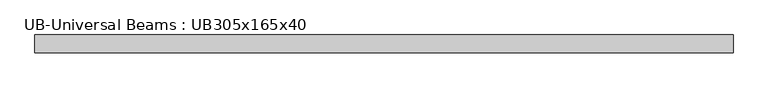
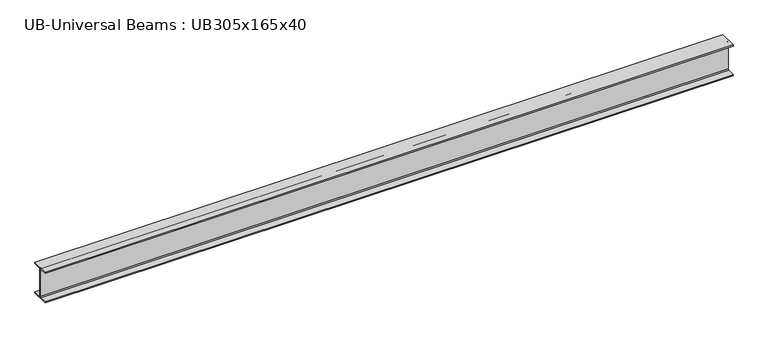
"""IFC4 building model written with IfcOpenShell, lengths in millimetres: beam geometry, UB-Universal Beams : UB305x165x40."""

import ifcopenshell
import ifcopenshell.guid

model = None  # the IFC model being written
_history = None  # IfcOwnerHistory: only IFC2X3 demands one
_inside = {}  # id of a spatial element -> (the spatial element, [elements in it])
_under = {}  # id of a project, library or spatial element -> (it, [spatial elements below it])
_declared = {}  # id of a project -> (the project, [libraries it declares])
_typed = {}  # id of a type object -> (the type object, [elements of that type])
_made_of = {}  # id of a material, layer set ... -> (it, [elements and type objects made of it])


def new_model(schema):
    """Start an empty IFC model of exactly this schema.

    Asked for "IFC4X3", IfcOpenShell would pick the latest addendum, in which some entities
    have other attributes; the version numbers below select the first issue.
    IFC2X3 requires an IfcOwnerHistory on every rooted entity: one is made here for all.
    """
    global model, _history
    if schema == "IFC4X3":
        model = ifcopenshell.file(schema_version=(4, 3, 0, 0))
    else:
        model = ifcopenshell.file(schema=schema)
    _inside.clear()
    _under.clear()
    _declared.clear()
    _typed.clear()
    _made_of.clear()
    _history = None
    if model.schema == "IFC2X3":
        org = make("IfcOrganization", Name="unknown")
        user = make(
            "IfcPersonAndOrganization",
            ThePerson=make("IfcPerson", FamilyName="unknown"),
            TheOrganization=org,
        )
        app = make(
            "IfcApplication",
            ApplicationDeveloper=org,
            Version="unknown",
            ApplicationFullName="unknown",
            ApplicationIdentifier="unknown",
        )
        _history = make(
            "IfcOwnerHistory",
            OwningUser=user,
            OwningApplication=app,
            ChangeAction="ADDED",
            CreationDate=0,
        )
    return model


def make(cls, **values):
    """One entity of the class cls with the attributes given. An attribute that is None is left unset."""
    return model.create_entity(
        cls, **{name: value for name, value in values.items() if value is not None}
    )


def rooted(cls, **values):
    """An entity with a GlobalId (a new one), such as an element, a storey or a relation."""
    return make(cls, GlobalId=ifcopenshell.guid.new(), OwnerHistory=_history, **values)


def si_unit(unit_type, name, prefix=None):
    """IfcSIUnit, for example si_unit("LENGTHUNIT", "METRE", prefix="MILLI")."""
    return make("IfcSIUnit", UnitType=unit_type, Prefix=prefix, Name=name)


def assignment(units):
    """IfcUnitAssignment: the units of a project."""
    return None if units is None else make("IfcUnitAssignment", Units=units)


def point(xyz):
    """IfcCartesianPoint."""
    return None if xyz is None else make("IfcCartesianPoint", Coordinates=xyz)


def direction(xyz):
    """IfcDirection."""
    return None if xyz is None else make("IfcDirection", DirectionRatios=xyz)


def frame(location, z_axis=None, x_axis=None):
    """IfcAxis2Placement3D, a coordinate frame: its origin and axes. An axis left out is left unset."""
    return make(
        "IfcAxis2Placement3D",
        Location=point(location),
        Axis=direction(z_axis),
        RefDirection=direction(x_axis),
    )


def frame_2d(location, x_axis=None):
    """IfcAxis2Placement2D, a coordinate frame in the plane: its origin and x axis."""
    return make(
        "IfcAxis2Placement2D", Location=point(location), RefDirection=direction(x_axis)
    )


def origin():
    """The frame at (0, 0, 0) with its axes left unset."""
    return frame((0.0, 0.0, 0.0))


def place(relative_to, where):
    """IfcLocalPlacement: puts the frame where relative to a parent placement (None: the world)."""
    return make(
        "IfcLocalPlacement", PlacementRelTo=relative_to, RelativePlacement=where
    )


def context(
    kind, dimensions, precision=None, world=None, true_north=None, identifier=None
):
    """IfcGeometricRepresentationContext, for example the 3D "Model" context."""
    return make(
        "IfcGeometricRepresentationContext",
        ContextIdentifier=identifier,
        ContextType=kind,
        CoordinateSpaceDimension=dimensions,
        Precision=precision,
        WorldCoordinateSystem=world,
        TrueNorth=true_north,
    )


def project(units=None, contexts=None):
    """IfcProject with its units and contexts."""
    return rooted(
        "IfcProject",
        Name="project",
        RepresentationContexts=contexts,
        UnitsInContext=assignment(units),
    )


def spatial(cls, under=None, at=None, **own):
    """A site, building, storey or space (cls), placed at a placement, below another one or the project."""
    s = rooted(cls, ObjectPlacement=at, **own)
    if under is not None:
        _under.setdefault(under.id(), (under, []))[1].append(s)
    return s


def polyline(points):
    """IfcPolyline through the points."""
    return make("IfcPolyline", Points=[point(p) for p in points])


def circle_curve(where, radius):
    """IfcCircle in the frame where."""
    return make("IfcCircle", Position=where, Radius=radius)


def trimmed(basis, trim1, trim2, sense, master):
    """IfcTrimmedCurve: the piece of a basis curve between two trims."""
    return make(
        "IfcTrimmedCurve",
        BasisCurve=basis,
        Trim1=trim1,
        Trim2=trim2,
        SenseAgreement=sense,
        MasterRepresentation=master,
    )


def segment(curve, same_sense, transition):
    """IfcCompositeCurveSegment."""
    return make(
        "IfcCompositeCurveSegment",
        Transition=transition,
        SameSense=same_sense,
        ParentCurve=curve,
    )


def composite_curve(segments, self_intersect=None):
    """IfcCompositeCurve: segments joined end to end."""
    return make("IfcCompositeCurve", Segments=segments, SelfIntersect=self_intersect)


def outline(outer, holes=None, kind="AREA"):
    """IfcArbitraryClosedProfileDef: a profile drawn as a closed curve; with holes, ...WithVoids."""
    if holes is None:
        return make("IfcArbitraryClosedProfileDef", ProfileType=kind, OuterCurve=outer)
    return make(
        "IfcArbitraryProfileDefWithVoids",
        ProfileType=kind,
        OuterCurve=outer,
        InnerCurves=holes,
    )


def extrude(swept, where, along, depth):
    """IfcExtrudedAreaSolid: the profile swept, set in the frame where, extruded along a direction by depth."""
    return make(
        "IfcExtrudedAreaSolid",
        SweptArea=swept,
        Position=where,
        ExtrudedDirection=direction(along),
        Depth=depth,
    )


def shape(context_of_items, identifier, shape_type, items):
    """IfcShapeRepresentation: the items that make up one representation, for example the "Body"."""
    return make(
        "IfcShapeRepresentation",
        ContextOfItems=context_of_items,
        RepresentationIdentifier=identifier,
        RepresentationType=shape_type,
        Items=items,
    )


def source(mapping_origin, context_of_items, identifier, shape_type, items):
    """IfcRepresentationMap: a shape defined once, which mapped items show again and again."""
    return make(
        "IfcRepresentationMap",
        MappingOrigin=mapping_origin,
        MappedRepresentation=shape(context_of_items, identifier, shape_type, items),
    )


def transform(
    local_origin,
    x_axis=None,
    y_axis=None,
    z_axis=None,
    scale=None,
    scale2=None,
    scale3=None,
    uniform=True,
):
    """IfcCartesianTransformationOperator3D, or its non-uniform kind. x_axis, y_axis, z_axis: its Axis1, 2, 3."""
    if uniform:
        return make(
            "IfcCartesianTransformationOperator3D",
            Axis1=direction(x_axis),
            Axis2=direction(y_axis),
            LocalOrigin=point(local_origin),
            Scale=scale,
            Axis3=direction(z_axis),
        )
    return make(
        "IfcCartesianTransformationOperator3DnonUniform",
        Axis1=direction(x_axis),
        Axis2=direction(y_axis),
        LocalOrigin=point(local_origin),
        Scale=scale,
        Axis3=direction(z_axis),
        Scale2=scale2,
        Scale3=scale3,
    )


def mapped(mapping_source, mapping_target):
    """IfcMappedItem: shows the shape of a source again, moved by a transform."""
    return make(
        "IfcMappedItem", MappingSource=mapping_source, MappingTarget=mapping_target
    )


def made_of(thing, what):
    """Note that an element or type object is made of a material, layer set ...; save() writes the relation."""
    if what is not None:
        _made_of.setdefault(what.id(), (what, []))[1].append(thing)
    return thing


def element(
    cls,
    number,
    at=None,
    inside=None,
    cuts=None,
    type_object=None,
    material=None,
    context=None,
    identifier="Body",
    shape_type=None,
    held_by="IfcProductDefinitionShape",
    body=None,
    shapes=None,
    **own,
):
    """One element of the class cls, such as IfcWall. Its Tag is "e" and its number.

    at: its placement. inside: the storey or other place that contains it. cuts: it is an
    opening in that element (IfcRelVoidsElement). A single representation is given by context,
    identifier, shape_type and body (its items); several are given by shapes. held_by: the class
    of the entity that holds the representations. save() writes the other relations.
    """
    e = rooted(cls, Tag="e%d" % number, ObjectPlacement=at, **own)
    if body is not None:
        shapes = [shape(context, identifier, shape_type, body)]
    if shapes is not None:
        e.Representation = make(held_by, Representations=shapes)
    if inside is not None:
        _inside.setdefault(inside.id(), (inside, []))[1].append(e)
    if cuts is not None:
        rooted(
            "IfcRelVoidsElement", RelatingBuildingElement=cuts, RelatedOpeningElement=e
        )
    if type_object is not None:
        _typed.setdefault(type_object.id(), (type_object, []))[1].append(e)
    return made_of(e, material)


def aggregate(whole, parts):
    """IfcRelAggregates: a whole, such as a stair, and the parts it consists of."""
    return rooted("IfcRelAggregates", RelatingObject=whole, RelatedObjects=parts)


def save(model, path):
    """Write the relations noted so far, then the file.

    IfcRelAggregates (storeys below a building ...), IfcRelContainedInSpatialStructure (elements
    in a storey), IfcRelDefinesByType, IfcRelAssociatesMaterial and IfcRelDeclares: one each for
    every whole, place, type object, material and project.
    """
    for whole, parts in _under.values():
        aggregate(whole, parts)
    for where, things in _inside.values():
        rooted(
            "IfcRelContainedInSpatialStructure",
            RelatedElements=things,
            RelatingStructure=where,
        )
    for kind, things in _typed.values():
        rooted("IfcRelDefinesByType", RelatedObjects=things, RelatingType=kind)
    for what, things in _made_of.values():
        rooted("IfcRelAssociatesMaterial", RelatedObjects=things, RelatingMaterial=what)
    for by, libraries in _declared.values():
        rooted("IfcRelDeclares", RelatingContext=by, RelatedDefinitions=libraries)
    model.write(path)


def ub_universal_beams_ub305x165x40_614cc3fe(model_context):
    return source(origin(), model_context, "Body", "SweptSolid", [
        extrude(outline(composite_curve([segment(polyline([(82.5, -141.5), (82.5, -151.7), (-82.5, -151.7), (-82.5, -141.5), (-11.9, -141.5)]), True, "CONTINUOUS"), segment(trimmed(circle_curve(frame_2d((-11.9, -132.6)), 8.9), [point((-11.9, -141.5))], [point((-3.0, -132.6))], True, "CARTESIAN"), True, "CONTINUOUS"), segment(polyline([(-3.0, -132.6), (-3.0, 132.6)]), True, "CONTINUOUS"), segment(trimmed(circle_curve(frame_2d((-11.9, 132.6)), 8.9), [point((-3.0, 132.6))], [point((-11.9, 141.5))], True, "CARTESIAN"), True, "CONTINUOUS"), segment(polyline([(-11.9, 141.5), (-82.5, 141.5), (-82.5, 151.7), (82.5, 151.7), (82.5, 141.5), (11.9, 141.5)]), True, "CONTINUOUS"), segment(trimmed(circle_curve(frame_2d((11.9, 132.6)), 8.9), [point((11.9, 141.5))], [point((3.0, 132.6))], True, "CARTESIAN"), True, "CONTINUOUS"), segment(polyline([(3.0, 132.6), (3.0, -132.6)]), True, "CONTINUOUS"), segment(trimmed(circle_curve(frame_2d((11.9, -132.6)), 8.9), [point((3.0, -132.6))], [point((11.9, -141.5))], True, "CARTESIAN"), True, "CONTINUOUS"), segment(polyline([(11.9, -141.5), (82.5, -141.5)]), True, "CONTINUOUS")], self_intersect=False)), frame((-3226.45, 0.0, 0.0), z_axis=(1.0, 0.0, 0.0), x_axis=(0.0, 1.0, 0.0)), (0.0, 0.0, 1.0), 6452.9),
    ])


if __name__ == "__main__":
    model = new_model("IFC4")
    model_context = context("Model", 3, world=origin())
    ifc_project = project(units=[si_unit("LENGTHUNIT", "METRE", prefix="MILLI")], contexts=[model_context])
    site = spatial("IfcSite", under=ifc_project)
    building = spatial("IfcBuilding", under=site)
    placement = place(None, origin())
    ub_universal_beams_ub305x165x40_shape = ub_universal_beams_ub305x165x40_614cc3fe(model_context)
    element("IfcBeam", 1, ObjectType="UB-Universal Beams : UB305x165x40", at=placement, inside=building, context=model_context, shape_type="MappedRepresentation", body=[
        mapped(ub_universal_beams_ub305x165x40_shape, transform((0.0, 0.0, 0.0), x_axis=(1.0, 0.0, 0.0), y_axis=(0.0, 1.0, 0.0), z_axis=(0.0, 0.0, 1.0))),
    ])
    save(model, "model.ifc")

# Revit data of these elements
# Type "UB-Universal Beams : UB305x165x40"
#   Section Name Key = "UB305X165X40"
#   Width = 16.5 cm
#   Web Thickness = 0.6 cm
#   Web Fillet = 0.89 cm
#   Warping Constant = 164000.0 cm⁶
#   Torsional Moment of Inertia = 14.70 cm⁴
#   Section Area = 51.3 cm²
#   Plastic Modulus weak axis = 142.0 cm³
#   Plastic Modulus strong axis = 623.0 cm³
#   Nominal Weight = 40.2999 kgf/m
#   Moment of Inertia weak axis = 764.00 cm⁴
#   Moment of Inertia strong axis = 8503.00 cm⁴
#   Height = 30.34 cm
#   Flange Thickness = 1.02 cm
#   Elastic Modulus weak axis = 92.6 cm³
#   Elastic Modulus strong axis = 560.0 cm³
#   Centroid Vertical = 15.17 cm
#   Centroid Horizontal = 8.25 cm
#   Bolt Spacing = 9.0 cm
#   Length [instance default] = 1500 mm
#   Structural Material [instance default] = Metal - Steel 43-275
#   Type Comments = ""
#   Assembly Code = ""
# Element 1 (IfcBeam, "UB-Universal Beams : UB305x165x40")
#   Materials on its faces: "Metal - Steel 43-275"
# Materials
#   "Metal - Steel 43-275": class "Metal", colour RGB 247 247 247, transparency 0, Cost = 0
